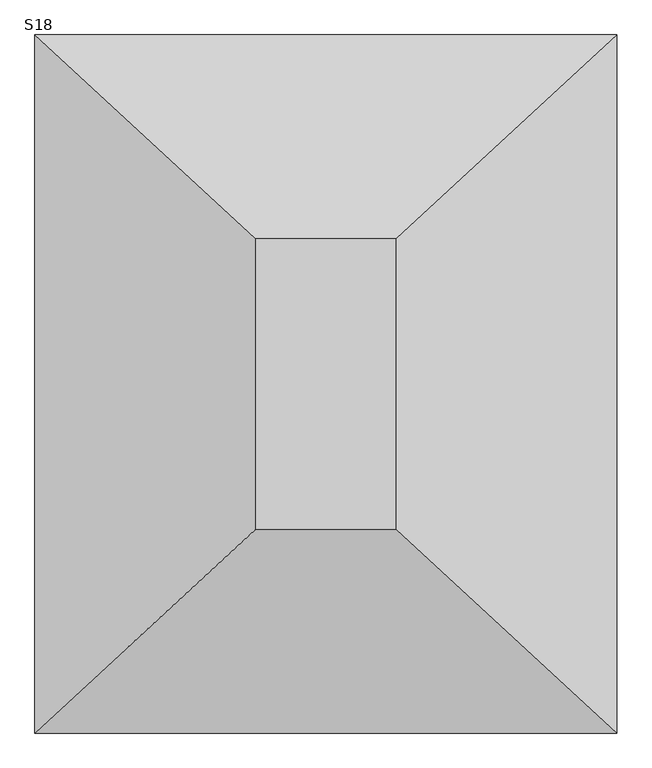
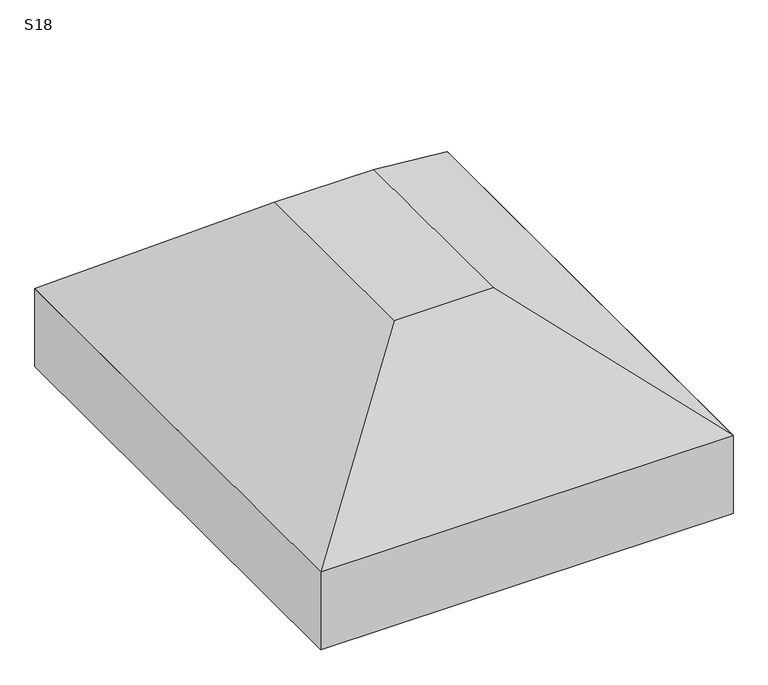
"""IFC4 building model written with IfcOpenShell, lengths in millimetres: fastener geometry, TQS - Sapata : S18."""

import ifcopenshell
import ifcopenshell.guid

model = None  # the IFC model being written
_history = None  # IfcOwnerHistory: only IFC2X3 demands one
_inside = {}  # id of a spatial element -> (the spatial element, [elements in it])
_under = {}  # id of a project, library or spatial element -> (it, [spatial elements below it])
_declared = {}  # id of a project -> (the project, [libraries it declares])
_typed = {}  # id of a type object -> (the type object, [elements of that type])
_made_of = {}  # id of a material, layer set ... -> (it, [elements and type objects made of it])


def new_model(schema):
    """Start an empty IFC model of exactly this schema.

    Asked for "IFC4X3", IfcOpenShell would pick the latest addendum, in which some entities
    have other attributes; the version numbers below select the first issue.
    IFC2X3 requires an IfcOwnerHistory on every rooted entity: one is made here for all.
    """
    global model, _history
    if schema == "IFC4X3":
        model = ifcopenshell.file(schema_version=(4, 3, 0, 0))
    else:
        model = ifcopenshell.file(schema=schema)
    _inside.clear()
    _under.clear()
    _declared.clear()
    _typed.clear()
    _made_of.clear()
    _history = None
    if model.schema == "IFC2X3":
        org = make("IfcOrganization", Name="unknown")
        user = make(
            "IfcPersonAndOrganization",
            ThePerson=make("IfcPerson", FamilyName="unknown"),
            TheOrganization=org,
        )
        app = make(
            "IfcApplication",
            ApplicationDeveloper=org,
            Version="unknown",
            ApplicationFullName="unknown",
            ApplicationIdentifier="unknown",
        )
        _history = make(
            "IfcOwnerHistory",
            OwningUser=user,
            OwningApplication=app,
            ChangeAction="ADDED",
            CreationDate=0,
        )
    return model


def make(cls, **values):
    """One entity of the class cls with the attributes given. An attribute that is None is left unset."""
    return model.create_entity(
        cls, **{name: value for name, value in values.items() if value is not None}
    )


def rooted(cls, **values):
    """An entity with a GlobalId (a new one), such as an element, a storey or a relation."""
    return make(cls, GlobalId=ifcopenshell.guid.new(), OwnerHistory=_history, **values)


def si_unit(unit_type, name, prefix=None):
    """IfcSIUnit, for example si_unit("LENGTHUNIT", "METRE", prefix="MILLI")."""
    return make("IfcSIUnit", UnitType=unit_type, Prefix=prefix, Name=name)


def assignment(units):
    """IfcUnitAssignment: the units of a project."""
    return None if units is None else make("IfcUnitAssignment", Units=units)


def point(xyz):
    """IfcCartesianPoint."""
    return None if xyz is None else make("IfcCartesianPoint", Coordinates=xyz)


def direction(xyz):
    """IfcDirection."""
    return None if xyz is None else make("IfcDirection", DirectionRatios=xyz)


def frame(location, z_axis=None, x_axis=None):
    """IfcAxis2Placement3D, a coordinate frame: its origin and axes. An axis left out is left unset."""
    return make(
        "IfcAxis2Placement3D",
        Location=point(location),
        Axis=direction(z_axis),
        RefDirection=direction(x_axis),
    )


def origin():
    """The frame at (0, 0, 0) with its axes left unset."""
    return frame((0.0, 0.0, 0.0))


def place(relative_to, where):
    """IfcLocalPlacement: puts the frame where relative to a parent placement (None: the world)."""
    return make(
        "IfcLocalPlacement", PlacementRelTo=relative_to, RelativePlacement=where
    )


def context(
    kind, dimensions, precision=None, world=None, true_north=None, identifier=None
):
    """IfcGeometricRepresentationContext, for example the 3D "Model" context."""
    return make(
        "IfcGeometricRepresentationContext",
        ContextIdentifier=identifier,
        ContextType=kind,
        CoordinateSpaceDimension=dimensions,
        Precision=precision,
        WorldCoordinateSystem=world,
        TrueNorth=true_north,
    )


def project(units=None, contexts=None):
    """IfcProject with its units and contexts."""
    return rooted(
        "IfcProject",
        Name="project",
        RepresentationContexts=contexts,
        UnitsInContext=assignment(units),
    )


def spatial(cls, under=None, at=None, **own):
    """A site, building, storey or space (cls), placed at a placement, below another one or the project."""
    s = rooted(cls, ObjectPlacement=at, **own)
    if under is not None:
        _under.setdefault(under.id(), (under, []))[1].append(s)
    return s


def polyline(points):
    """IfcPolyline through the points."""
    return make("IfcPolyline", Points=[point(p) for p in points])


def outline(outer, holes=None, kind="AREA"):
    """IfcArbitraryClosedProfileDef: a profile drawn as a closed curve; with holes, ...WithVoids."""
    if holes is None:
        return make("IfcArbitraryClosedProfileDef", ProfileType=kind, OuterCurve=outer)
    return make(
        "IfcArbitraryProfileDefWithVoids",
        ProfileType=kind,
        OuterCurve=outer,
        InnerCurves=holes,
    )


def extrude(swept, where, along, depth):
    """IfcExtrudedAreaSolid: the profile swept, set in the frame where, extruded along a direction by depth."""
    return make(
        "IfcExtrudedAreaSolid",
        SweptArea=swept,
        Position=where,
        ExtrudedDirection=direction(along),
        Depth=depth,
    )


def faces_of(points, faces, orient=None, outer=None):
    """IfcFace entities. A face is a list of loops; a loop is a list of indices into points, from 0.

    orient and outer hold one flag for each loop. By default every Orientation is true, the
    first loop of a face is its IfcFaceOuterBound and the others are IfcFaceBound.
    """
    made = []
    for i, loops in enumerate(faces):
        bounds = []
        for j, loop in enumerate(loops):
            is_outer = j == 0 if outer is None else outer[i][j]
            bounds.append(
                make(
                    "IfcFaceOuterBound" if is_outer else "IfcFaceBound",
                    Bound=make("IfcPolyLoop", Polygon=[points[k] for k in loop]),
                    Orientation=True if orient is None else orient[i][j],
                )
            )
        made.append(make("IfcFace", Bounds=bounds))
    return made


def faceted_brep(points, faces, orient=None, outer=None, voids=None):
    """IfcFacetedBrep: a solid bounded by flat faces; with voids (closed shells), ...WithVoids."""
    shared = [point(p) for p in points]
    hull = make("IfcClosedShell", CfsFaces=faces_of(shared, faces, orient, outer))
    if voids is None:
        return make("IfcFacetedBrep", Outer=hull)
    return make(
        "IfcFacetedBrepWithVoids",
        Outer=hull,
        Voids=[
            make(cls, CfsFaces=faces_of(shared, fs, o, b)) for cls, fs, o, b in voids
        ],
    )


def shape(context_of_items, identifier, shape_type, items):
    """IfcShapeRepresentation: the items that make up one representation, for example the "Body"."""
    return make(
        "IfcShapeRepresentation",
        ContextOfItems=context_of_items,
        RepresentationIdentifier=identifier,
        RepresentationType=shape_type,
        Items=items,
    )


def source(mapping_origin, context_of_items, identifier, shape_type, items):
    """IfcRepresentationMap: a shape defined once, which mapped items show again and again."""
    return make(
        "IfcRepresentationMap",
        MappingOrigin=mapping_origin,
        MappedRepresentation=shape(context_of_items, identifier, shape_type, items),
    )


def transform(
    local_origin,
    x_axis=None,
    y_axis=None,
    z_axis=None,
    scale=None,
    scale2=None,
    scale3=None,
    uniform=True,
):
    """IfcCartesianTransformationOperator3D, or its non-uniform kind. x_axis, y_axis, z_axis: its Axis1, 2, 3."""
    if uniform:
        return make(
            "IfcCartesianTransformationOperator3D",
            Axis1=direction(x_axis),
            Axis2=direction(y_axis),
            LocalOrigin=point(local_origin),
            Scale=scale,
            Axis3=direction(z_axis),
        )
    return make(
        "IfcCartesianTransformationOperator3DnonUniform",
        Axis1=direction(x_axis),
        Axis2=direction(y_axis),
        LocalOrigin=point(local_origin),
        Scale=scale,
        Axis3=direction(z_axis),
        Scale2=scale2,
        Scale3=scale3,
    )


def mapped(mapping_source, mapping_target):
    """IfcMappedItem: shows the shape of a source again, moved by a transform."""
    return make(
        "IfcMappedItem", MappingSource=mapping_source, MappingTarget=mapping_target
    )


def made_of(thing, what):
    """Note that an element or type object is made of a material, layer set ...; save() writes the relation."""
    if what is not None:
        _made_of.setdefault(what.id(), (what, []))[1].append(thing)
    return thing


def element(
    cls,
    number,
    at=None,
    inside=None,
    cuts=None,
    type_object=None,
    material=None,
    context=None,
    identifier="Body",
    shape_type=None,
    held_by="IfcProductDefinitionShape",
    body=None,
    shapes=None,
    **own,
):
    """One element of the class cls, such as IfcWall. Its Tag is "e" and its number.

    at: its placement. inside: the storey or other place that contains it. cuts: it is an
    opening in that element (IfcRelVoidsElement). A single representation is given by context,
    identifier, shape_type and body (its items); several are given by shapes. held_by: the class
    of the entity that holds the representations. save() writes the other relations.
    """
    e = rooted(cls, Tag="e%d" % number, ObjectPlacement=at, **own)
    if body is not None:
        shapes = [shape(context, identifier, shape_type, body)]
    if shapes is not None:
        e.Representation = make(held_by, Representations=shapes)
    if inside is not None:
        _inside.setdefault(inside.id(), (inside, []))[1].append(e)
    if cuts is not None:
        rooted(
            "IfcRelVoidsElement", RelatingBuildingElement=cuts, RelatedOpeningElement=e
        )
    if type_object is not None:
        _typed.setdefault(type_object.id(), (type_object, []))[1].append(e)
    return made_of(e, material)


def aggregate(whole, parts):
    """IfcRelAggregates: a whole, such as a stair, and the parts it consists of."""
    return rooted("IfcRelAggregates", RelatingObject=whole, RelatedObjects=parts)


def save(model, path):
    """Write the relations noted so far, then the file.

    IfcRelAggregates (storeys below a building ...), IfcRelContainedInSpatialStructure (elements
    in a storey), IfcRelDefinesByType, IfcRelAssociatesMaterial and IfcRelDeclares: one each for
    every whole, place, type object, material and project.
    """
    for whole, parts in _under.values():
        aggregate(whole, parts)
    for where, things in _inside.values():
        rooted(
            "IfcRelContainedInSpatialStructure",
            RelatedElements=things,
            RelatingStructure=where,
        )
    for kind, things in _typed.values():
        rooted("IfcRelDefinesByType", RelatedObjects=things, RelatingType=kind)
    for what, things in _made_of.values():
        rooted("IfcRelAssociatesMaterial", RelatedObjects=things, RelatingMaterial=what)
    for by, libraries in _declared.values():
        rooted("IfcRelDeclares", RelatingContext=by, RelatedDefinitions=libraries)
    model.write(path)


def s18_084f9c6a(model_context):
    return source(origin(), model_context, "Body", "SolidModel", [
        faceted_brep([(-80.0, 50.0, 0.0), (-320.0, 50.0, 0.0), (-320.0, -450.0, 0.0), (-80.0, -450.0, 0.0), (300.0, 400.0, -300.0), (300.0, -800.0, -300.0), (-700.0, -800.0, -300.0), (-700.0, 400.0, -300.0)], [[[0, 1, 2, 3]], [[4, 5, 6, 7]], [[4, 7, 1, 0]], [[7, 6, 2, 1]], [[6, 5, 3, 2]], [[5, 4, 0, 3]]]),
        extrude(outline(polyline([(300.0, 400.0), (300.0, -800.0), (-700.0, -800.0), (-700.0, 400.0), (300.0, 400.0)])), frame((0.0, 0.0, -500.0), z_axis=(0.0, 0.0, 1.0), x_axis=(1.0, 0.0, 0.0)), (0.0, 0.0, 1.0), 200.0),
    ])


if __name__ == "__main__":
    model = new_model("IFC4")
    model_context = context("Model", 3, world=origin())
    ifc_project = project(units=[si_unit("LENGTHUNIT", "METRE", prefix="MILLI")], contexts=[model_context])
    site = spatial("IfcSite", under=ifc_project)
    building = spatial("IfcBuilding", under=site)
    placement = place(None, origin())
    s18_shape = s18_084f9c6a(model_context)
    element("IfcFastener", 1, ObjectType="TQS - Sapata : S18", at=placement, inside=building, context=model_context, shape_type="MappedRepresentation", body=[
        mapped(s18_shape, transform((0.0, 0.0, 0.0), x_axis=(1.0, 0.0, 0.0), y_axis=(0.0, 1.0, 0.0), z_axis=(0.0, 0.0, 1.0))),
    ])
    save(model, "model.ifc")

# Revit data of these elements
# Type "TQS - Sapata : S18"
#   TY = 0.50 m
#   TX = 0.24 m
#   HS = 0.50 m
#   H0 = 0.20 m
#   EXCYABS = 0.60 m
#   EXCY = 0.00 m
#   EXCXABS = 0.50 m
#   EXCX = 0.00 m
#   DIMY = 1.20 m
#   DIMX = 1.00 m
#   Material estrutural = Concreto - Concreto concretado no local
#   Width = 0
#   Length = 0
# Element 1 (IfcFastener, "TQS - Sapata : S18")
#   Materials on its faces: "Concreto - Concreto concretado no local"
# Materials
#   "Concreto - Concreto concretado no local": class "Concreto", colour RGB 192 192 192, transparency 0
